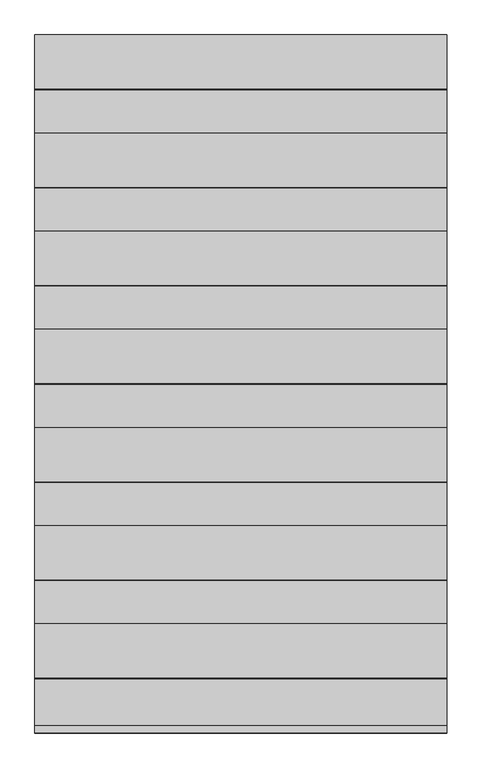
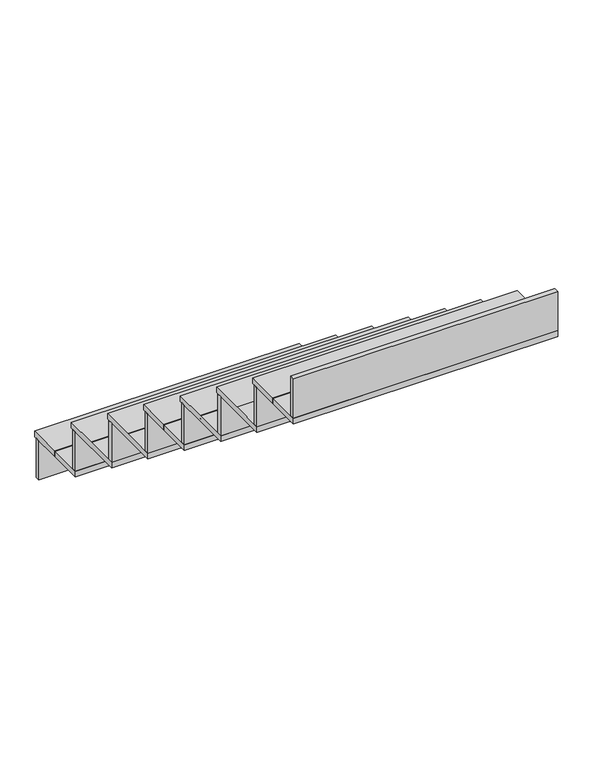
"""IFC4 building model written with IfcOpenShell, lengths in millimetres: stair flight geometry."""

from ifc_helpers import new_model, si_unit, frame, origin, place, context, project, spatial, polyline, outline, extrude, source, transform, mapped, element, save


def stair_flight_8e667a80(model_context):
    return source(origin(), model_context, "Body", "SweptSolid", [
        extrude(outline(polyline([(-23943.9164763, -9473.4570712), (-23943.9164763, -9454.4070712), (-22877.1164763, -9454.4070712), (-22877.1164763, -9473.4570712), (-23943.9164763, -9473.4570712)])), frame((0.0, 0.0, 1342.39), z_axis=(0.0, 0.0, 1.0), x_axis=(1.0, 0.0, 0.0)), (0.0, 0.0, 1.0), 167.8582813),
        extrude(outline(polyline([(-9584.5820712, 1510.2482813), (-9584.5820712, 1522.0025533), (-9587.7570712, 1522.0025533), (-9587.7570712, 1510.2482812), (-9727.4570712, 1510.2482812), (-9727.4570712, 1534.16), (-9587.7570712, 1534.16), (-9587.7570712, 1522.4057279), (-9584.5820712, 1522.4057279), (-9584.5820712, 1534.16), (-9444.8820712, 1534.16), (-9444.8820712, 1510.2482813), (-9584.5820712, 1510.2482813)])), frame((-23943.9164763, 0.0, 0.0), z_axis=(1.0, 0.0, 0.0), x_axis=(0.0, 1.0, 0.0)), (0.0, 0.0, 1.0), 1066.8),
        extrude(outline(polyline([(-23943.9164763, -9727.4570712), (-23943.9164763, -9708.4070712), (-22877.1164763, -9708.4070712), (-22877.1164763, -9727.4570712), (-23943.9164763, -9727.4570712)])), frame((0.0, 0.0, 1534.16), z_axis=(0.0, 0.0, 1.0), x_axis=(1.0, 0.0, 0.0)), (0.0, 0.0, 1.0), 167.8582812),
        extrude(outline(polyline([(-9838.5820712, 1702.0182812), (-9838.5820712, 1713.7725533), (-9841.7570712, 1713.7725533), (-9841.7570712, 1702.0182812), (-9981.4570712, 1702.0182812), (-9981.4570712, 1725.93), (-9841.7570712, 1725.93), (-9841.7570712, 1714.1757279), (-9838.5820712, 1714.1757279), (-9838.5820712, 1725.93), (-9698.8820712, 1725.93), (-9698.8820712, 1702.0182812), (-9838.5820712, 1702.0182812)])), frame((-23943.9164763, 0.0, 0.0), z_axis=(1.0, 0.0, 0.0), x_axis=(0.0, 1.0, 0.0)), (0.0, 0.0, 1.0), 1066.8),
        extrude(outline(polyline([(-23943.9164763, -9981.4570712), (-23943.9164763, -9962.4070712), (-22877.1164763, -9962.4070712), (-22877.1164763, -9981.4570712), (-23943.9164763, -9981.4570712)])), frame((0.0, 0.0, 1725.93), z_axis=(0.0, 0.0, 1.0), x_axis=(1.0, 0.0, 0.0)), (0.0, 0.0, 1.0), 167.8582812),
        extrude(outline(polyline([(-10092.5820712, 1893.7882813), (-10092.5820712, 1905.5425533), (-10095.7570712, 1905.5425533), (-10095.7570712, 1893.7882812), (-10235.4570712, 1893.7882812), (-10235.4570712, 1917.7), (-10095.7570712, 1917.7), (-10095.7570712, 1905.9457279), (-10092.5820712, 1905.9457279), (-10092.5820712, 1917.7), (-9952.8820712, 1917.7), (-9952.8820712, 1893.7882813), (-10092.5820712, 1893.7882813)])), frame((-23943.9164763, 0.0, 0.0), z_axis=(1.0, 0.0, 0.0), x_axis=(0.0, 1.0, 0.0)), (0.0, 0.0, 1.0), 1066.8),
        extrude(outline(polyline([(-23943.9164763, -10235.4570712), (-23943.9164763, -10216.4070712), (-22877.1164763, -10216.4070712), (-22877.1164763, -10235.4570712), (-23943.9164763, -10235.4570712)])), frame((0.0, 0.0, 1917.7), z_axis=(0.0, 0.0, 1.0), x_axis=(1.0, 0.0, 0.0)), (0.0, 0.0, 1.0), 167.8582812),
        extrude(outline(polyline([(-10346.5820712, 2085.5582813), (-10346.5820712, 2097.3125533), (-10349.7570712, 2097.3125533), (-10349.7570712, 2085.5582812), (-10489.4570712, 2085.5582812), (-10489.4570712, 2109.47), (-10349.7570712, 2109.47), (-10349.7570712, 2097.7157279), (-10346.5820712, 2097.7157279), (-10346.5820712, 2109.47), (-10206.8820712, 2109.47), (-10206.8820712, 2085.5582813), (-10346.5820712, 2085.5582813)])), frame((-23943.9164763, 0.0, 0.0), z_axis=(1.0, 0.0, 0.0), x_axis=(0.0, 1.0, 0.0)), (0.0, 0.0, 1.0), 1066.8),
        extrude(outline(polyline([(-23943.9164763, -10489.4570712), (-23943.9164763, -10470.4070712), (-22877.1164763, -10470.4070712), (-22877.1164763, -10489.4570712), (-23943.9164763, -10489.4570712)])), frame((0.0, 0.0, 2109.47), z_axis=(0.0, 0.0, 1.0), x_axis=(1.0, 0.0, 0.0)), (0.0, 0.0, 1.0), 167.8582812),
        extrude(outline(polyline([(-10600.5820712, 2277.3282813), (-10600.5820712, 2289.0825533), (-10603.7570712, 2289.0825533), (-10603.7570712, 2277.3282812), (-10743.4570712, 2277.3282812), (-10743.4570712, 2301.24), (-10603.7570712, 2301.24), (-10603.7570712, 2289.4857279), (-10600.5820712, 2289.4857279), (-10600.5820712, 2301.24), (-10460.8820712, 2301.24), (-10460.8820712, 2277.3282813), (-10600.5820712, 2277.3282813)])), frame((-23943.9164763, 0.0, 0.0), z_axis=(1.0, 0.0, 0.0), x_axis=(0.0, 1.0, 0.0)), (0.0, 0.0, 1.0), 1066.8),
        extrude(outline(polyline([(-23943.9164763, -10743.4570712), (-23943.9164763, -10724.4070712), (-22877.1164763, -10724.4070712), (-22877.1164763, -10743.4570712), (-23943.9164763, -10743.4570712)])), frame((0.0, 0.0, 2301.24), z_axis=(0.0, 0.0, 1.0), x_axis=(1.0, 0.0, 0.0)), (0.0, 0.0, 1.0), 167.8582812),
        extrude(outline(polyline([(-10854.5820712, 2469.0982813), (-10854.5820712, 2480.8525533), (-10857.7570712, 2480.8525533), (-10857.7570712, 2469.0982812), (-10997.4570712, 2469.0982812), (-10997.4570712, 2493.01), (-10857.7570712, 2493.01), (-10857.7570712, 2481.2557279), (-10854.5820712, 2481.2557279), (-10854.5820712, 2493.01), (-10714.8820712, 2493.01), (-10714.8820712, 2469.0982813), (-10854.5820712, 2469.0982813)])), frame((-23943.9164763, 0.0, 0.0), z_axis=(1.0, 0.0, 0.0), x_axis=(0.0, 1.0, 0.0)), (0.0, 0.0, 1.0), 1066.8),
        extrude(outline(polyline([(-23943.9164763, -10997.4570712), (-23943.9164763, -10978.4070712), (-22877.1164763, -10978.4070712), (-22877.1164763, -10997.4570712), (-23943.9164763, -10997.4570712)])), frame((0.0, 0.0, 2493.01), z_axis=(0.0, 0.0, 1.0), x_axis=(1.0, 0.0, 0.0)), (0.0, 0.0, 1.0), 167.8582812),
        extrude(outline(polyline([(-11108.5820712, 2660.8682813), (-11108.5820712, 2672.6225533), (-11111.7570712, 2672.6225533), (-11111.7570712, 2660.8682812), (-11251.4570712, 2660.8682812), (-11251.4570712, 2684.78), (-11111.7570712, 2684.78), (-11111.7570712, 2673.0257279), (-11108.5820712, 2673.0257279), (-11108.5820712, 2684.78), (-10968.8820712, 2684.78), (-10968.8820712, 2660.8682813), (-11108.5820712, 2660.8682813)])), frame((-23943.9164763, 0.0, 0.0), z_axis=(1.0, 0.0, 0.0), x_axis=(0.0, 1.0, 0.0)), (0.0, 0.0, 1.0), 1066.8),
        extrude(outline(polyline([(-23943.9164763, -11251.4570712), (-23943.9164763, -11232.4070712), (-22877.1164763, -11232.4070712), (-22877.1164763, -11251.4570712), (-23943.9164763, -11251.4570712)])), frame((0.0, 0.0, 2684.78), z_axis=(0.0, 0.0, 1.0), x_axis=(1.0, 0.0, 0.0)), (0.0, 0.0, 1.0), 167.8582812),
    ])


if __name__ == "__main__":
    model = new_model("IFC4")
    model_context = context("Model", 3, world=origin())
    ifc_project = project(units=[si_unit("LENGTHUNIT", "METRE", prefix="MILLI")], contexts=[model_context])
    site = spatial("IfcSite", under=ifc_project)
    building = spatial("IfcBuilding", under=site)
    placement = place(None, origin())
    stair_flight_shape = stair_flight_8e667a80(model_context)
    element("IfcStairFlight", 1, at=placement, inside=building, context=model_context, shape_type="MappedRepresentation", body=[
        mapped(stair_flight_shape, transform((0.0, 0.0, 0.0), x_axis=(1.0, 0.0, 0.0), y_axis=(0.0, 1.0, 0.0), z_axis=(0.0, 0.0, 1.0))),
    ])
    save(model, "model.ifc")

# Revit data of these elements
# Element 1 (IfcStairFlight)
#   Materials on its faces: "DEFAULT DOOR"
# Materials
#   "DEFAULT DOOR": class "Generic", colour RGB 216 216 216, transparency 0, Cost = 0
